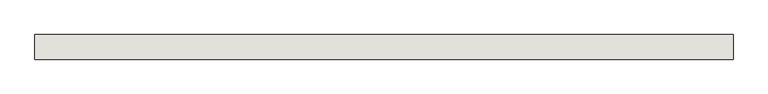
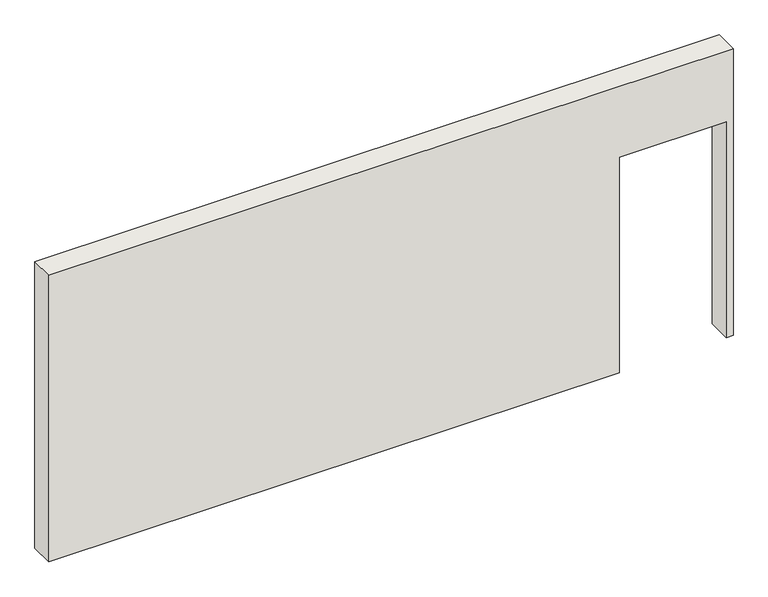
"""IFC4 building model written with IfcOpenShell, lengths in millimetres: wall geometry, Holzwand."""

import ifcopenshell
import ifcopenshell.guid

model = None  # the IFC model being written
_history = None  # IfcOwnerHistory: only IFC2X3 demands one
_inside = {}  # id of a spatial element -> (the spatial element, [elements in it])
_under = {}  # id of a project, library or spatial element -> (it, [spatial elements below it])
_declared = {}  # id of a project -> (the project, [libraries it declares])
_typed = {}  # id of a type object -> (the type object, [elements of that type])
_made_of = {}  # id of a material, layer set ... -> (it, [elements and type objects made of it])


def new_model(schema):
    """Start an empty IFC model of exactly this schema.

    Asked for "IFC4X3", IfcOpenShell would pick the latest addendum, in which some entities
    have other attributes; the version numbers below select the first issue.
    IFC2X3 requires an IfcOwnerHistory on every rooted entity: one is made here for all.
    """
    global model, _history
    if schema == "IFC4X3":
        model = ifcopenshell.file(schema_version=(4, 3, 0, 0))
    else:
        model = ifcopenshell.file(schema=schema)
    _inside.clear()
    _under.clear()
    _declared.clear()
    _typed.clear()
    _made_of.clear()
    _history = None
    if model.schema == "IFC2X3":
        org = make("IfcOrganization", Name="unknown")
        user = make(
            "IfcPersonAndOrganization",
            ThePerson=make("IfcPerson", FamilyName="unknown"),
            TheOrganization=org,
        )
        app = make(
            "IfcApplication",
            ApplicationDeveloper=org,
            Version="unknown",
            ApplicationFullName="unknown",
            ApplicationIdentifier="unknown",
        )
        _history = make(
            "IfcOwnerHistory",
            OwningUser=user,
            OwningApplication=app,
            ChangeAction="ADDED",
            CreationDate=0,
        )
    return model


def make(cls, **values):
    """One entity of the class cls with the attributes given. An attribute that is None is left unset."""
    return model.create_entity(
        cls, **{name: value for name, value in values.items() if value is not None}
    )


def rooted(cls, **values):
    """An entity with a GlobalId (a new one), such as an element, a storey or a relation."""
    return make(cls, GlobalId=ifcopenshell.guid.new(), OwnerHistory=_history, **values)


def si_unit(unit_type, name, prefix=None):
    """IfcSIUnit, for example si_unit("LENGTHUNIT", "METRE", prefix="MILLI")."""
    return make("IfcSIUnit", UnitType=unit_type, Prefix=prefix, Name=name)


def assignment(units):
    """IfcUnitAssignment: the units of a project."""
    return None if units is None else make("IfcUnitAssignment", Units=units)


def point(xyz):
    """IfcCartesianPoint."""
    return None if xyz is None else make("IfcCartesianPoint", Coordinates=xyz)


def direction(xyz):
    """IfcDirection."""
    return None if xyz is None else make("IfcDirection", DirectionRatios=xyz)


def frame(location, z_axis=None, x_axis=None):
    """IfcAxis2Placement3D, a coordinate frame: its origin and axes. An axis left out is left unset."""
    return make(
        "IfcAxis2Placement3D",
        Location=point(location),
        Axis=direction(z_axis),
        RefDirection=direction(x_axis),
    )


def origin():
    """The frame at (0, 0, 0) with its axes left unset."""
    return frame((0.0, 0.0, 0.0))


def place(relative_to, where):
    """IfcLocalPlacement: puts the frame where relative to a parent placement (None: the world)."""
    return make(
        "IfcLocalPlacement", PlacementRelTo=relative_to, RelativePlacement=where
    )


def context(
    kind, dimensions, precision=None, world=None, true_north=None, identifier=None
):
    """IfcGeometricRepresentationContext, for example the 3D "Model" context."""
    return make(
        "IfcGeometricRepresentationContext",
        ContextIdentifier=identifier,
        ContextType=kind,
        CoordinateSpaceDimension=dimensions,
        Precision=precision,
        WorldCoordinateSystem=world,
        TrueNorth=true_north,
    )


def project(units=None, contexts=None):
    """IfcProject with its units and contexts."""
    return rooted(
        "IfcProject",
        Name="project",
        RepresentationContexts=contexts,
        UnitsInContext=assignment(units),
    )


def spatial(cls, under=None, at=None, **own):
    """A site, building, storey or space (cls), placed at a placement, below another one or the project."""
    s = rooted(cls, ObjectPlacement=at, **own)
    if under is not None:
        _under.setdefault(under.id(), (under, []))[1].append(s)
    return s


def polyline(points):
    """IfcPolyline through the points."""
    return make("IfcPolyline", Points=[point(p) for p in points])


def outline(outer, holes=None, kind="AREA"):
    """IfcArbitraryClosedProfileDef: a profile drawn as a closed curve; with holes, ...WithVoids."""
    if holes is None:
        return make("IfcArbitraryClosedProfileDef", ProfileType=kind, OuterCurve=outer)
    return make(
        "IfcArbitraryProfileDefWithVoids",
        ProfileType=kind,
        OuterCurve=outer,
        InnerCurves=holes,
    )


def extrude(swept, where, along, depth):
    """IfcExtrudedAreaSolid: the profile swept, set in the frame where, extruded along a direction by depth."""
    return make(
        "IfcExtrudedAreaSolid",
        SweptArea=swept,
        Position=where,
        ExtrudedDirection=direction(along),
        Depth=depth,
    )


def shape(context_of_items, identifier, shape_type, items):
    """IfcShapeRepresentation: the items that make up one representation, for example the "Body"."""
    return make(
        "IfcShapeRepresentation",
        ContextOfItems=context_of_items,
        RepresentationIdentifier=identifier,
        RepresentationType=shape_type,
        Items=items,
    )


def source(mapping_origin, context_of_items, identifier, shape_type, items):
    """IfcRepresentationMap: a shape defined once, which mapped items show again and again."""
    return make(
        "IfcRepresentationMap",
        MappingOrigin=mapping_origin,
        MappedRepresentation=shape(context_of_items, identifier, shape_type, items),
    )


def transform(
    local_origin,
    x_axis=None,
    y_axis=None,
    z_axis=None,
    scale=None,
    scale2=None,
    scale3=None,
    uniform=True,
):
    """IfcCartesianTransformationOperator3D, or its non-uniform kind. x_axis, y_axis, z_axis: its Axis1, 2, 3."""
    if uniform:
        return make(
            "IfcCartesianTransformationOperator3D",
            Axis1=direction(x_axis),
            Axis2=direction(y_axis),
            LocalOrigin=point(local_origin),
            Scale=scale,
            Axis3=direction(z_axis),
        )
    return make(
        "IfcCartesianTransformationOperator3DnonUniform",
        Axis1=direction(x_axis),
        Axis2=direction(y_axis),
        LocalOrigin=point(local_origin),
        Scale=scale,
        Axis3=direction(z_axis),
        Scale2=scale2,
        Scale3=scale3,
    )


def mapped(mapping_source, mapping_target):
    """IfcMappedItem: shows the shape of a source again, moved by a transform."""
    return make(
        "IfcMappedItem", MappingSource=mapping_source, MappingTarget=mapping_target
    )


def made_of(thing, what):
    """Note that an element or type object is made of a material, layer set ...; save() writes the relation."""
    if what is not None:
        _made_of.setdefault(what.id(), (what, []))[1].append(thing)
    return thing


def element(
    cls,
    number,
    at=None,
    inside=None,
    cuts=None,
    type_object=None,
    material=None,
    context=None,
    identifier="Body",
    shape_type=None,
    held_by="IfcProductDefinitionShape",
    body=None,
    shapes=None,
    **own,
):
    """One element of the class cls, such as IfcWall. Its Tag is "e" and its number.

    at: its placement. inside: the storey or other place that contains it. cuts: it is an
    opening in that element (IfcRelVoidsElement). A single representation is given by context,
    identifier, shape_type and body (its items); several are given by shapes. held_by: the class
    of the entity that holds the representations. save() writes the other relations.
    """
    e = rooted(cls, Tag="e%d" % number, ObjectPlacement=at, **own)
    if body is not None:
        shapes = [shape(context, identifier, shape_type, body)]
    if shapes is not None:
        e.Representation = make(held_by, Representations=shapes)
    if inside is not None:
        _inside.setdefault(inside.id(), (inside, []))[1].append(e)
    if cuts is not None:
        rooted(
            "IfcRelVoidsElement", RelatingBuildingElement=cuts, RelatedOpeningElement=e
        )
    if type_object is not None:
        _typed.setdefault(type_object.id(), (type_object, []))[1].append(e)
    return made_of(e, material)


def aggregate(whole, parts):
    """IfcRelAggregates: a whole, such as a stair, and the parts it consists of."""
    return rooted("IfcRelAggregates", RelatingObject=whole, RelatedObjects=parts)


def save(model, path):
    """Write the relations noted so far, then the file.

    IfcRelAggregates (storeys below a building ...), IfcRelContainedInSpatialStructure (elements
    in a storey), IfcRelDefinesByType, IfcRelAssociatesMaterial and IfcRelDeclares: one each for
    every whole, place, type object, material and project.
    """
    for whole, parts in _under.values():
        aggregate(whole, parts)
    for where, things in _inside.values():
        rooted(
            "IfcRelContainedInSpatialStructure",
            RelatedElements=things,
            RelatingStructure=where,
        )
    for kind, things in _typed.values():
        rooted("IfcRelDefinesByType", RelatedObjects=things, RelatingType=kind)
    for what, things in _made_of.values():
        rooted("IfcRelAssociatesMaterial", RelatedObjects=things, RelatingMaterial=what)
    for by, libraries in _declared.values():
        rooted("IfcRelDeclares", RelatingContext=by, RelatedDefinitions=libraries)
    model.write(path)


def wall_c528e420(model_context):
    return source(origin(), model_context, "Body", "SweptSolid", [
        extrude(outline(polyline([(0.0, 4727.1048224), (1890.0, 4727.1048224), (1890.0, 5612.1048224), (0.0, 5612.1048224), (0.0, 5670.0), (2510.0, 5670.0), (2510.0, 0.0), (0.0, 0.0), (0.0, 4727.1048224)])), frame((0.0, 0.0, 0.0), z_axis=(0.0, 1.0, 0.0), x_axis=(0.0, 0.0, 1.0)), (0.0, 0.0, 1.0), 200.0),
    ])


if __name__ == "__main__":
    model = new_model("IFC4")
    model_context = context("Model", 3, world=origin())
    ifc_project = project(units=[si_unit("LENGTHUNIT", "METRE", prefix="MILLI")], contexts=[model_context])
    site = spatial("IfcSite", under=ifc_project)
    building = spatial("IfcBuilding", under=site)
    placement = place(None, origin())
    wall_shape = wall_c528e420(model_context)
    element("IfcWall", 1, ObjectType="Holzwand", at=placement, inside=building, context=model_context, shape_type="MappedRepresentation", body=[
        mapped(wall_shape, transform((0.0, 0.0, 0.0), x_axis=(1.0, 0.0, 0.0), y_axis=(0.0, 1.0, 0.0), z_axis=(0.0, 0.0, 1.0))),
    ])
    save(model, "model.ifc")

# Revit data of these elements
# Element 1 (IfcWall, "Holzwand")
#   Materials on its faces: "holzschalung"
# Materials
#   "holzschalung": class "Unassigned", colour RGB 128 128 128, transparency 0
